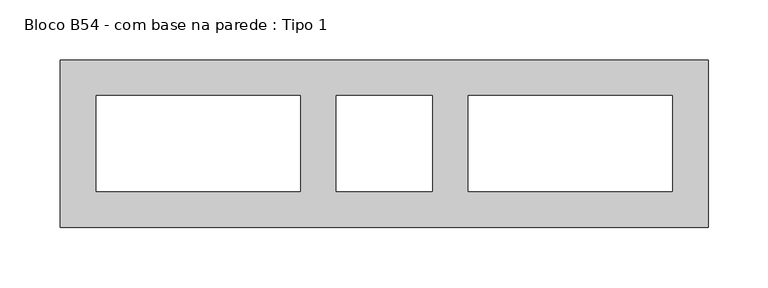
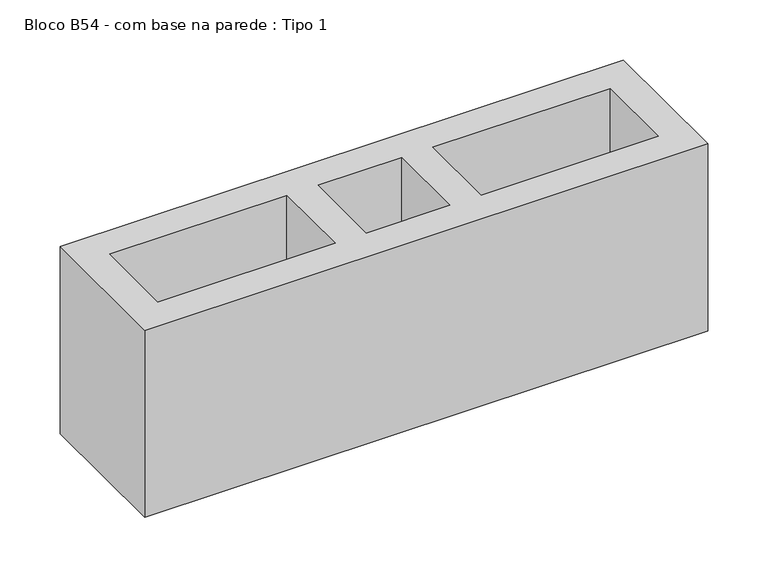
"""IFC4 building model written with IfcOpenShell, lengths in millimetres: proxy geometry, Bloco B54 - com base na parede : Tipo 1."""

from ifc_helpers import new_model, si_unit, origin, origin_with_axes, place, context, project, spatial, polyline, outline, extrude, source, transform, mapped, element, save


def bloco_b54_com_base_na_parede_tipo_1_bb8c27e4(model_context):
    return source(origin(), model_context, "Body", "SweptSolid", [
        extrude(outline(polyline([(320.0, -70.0), (-220.0, -70.0), (-220.0, 70.0), (320.0, 70.0), (320.0, -70.0)]), holes=[polyline([(120.0, -40.0), (290.0, -40.0), (290.0, 40.0), (120.0, 40.0), (120.0, -40.0)]), polyline([(-20.0, -40.0), (-20.0, 40.0), (-190.0, 40.0), (-190.0, -40.0), (-20.0, -40.0)]), polyline([(90.0, -40.0), (90.0, 40.0), (10.0, 40.0), (10.0, -40.0), (90.0, -40.0)])]), origin_with_axes(), (0.0, 0.0, 1.0), 190.0),
    ])


if __name__ == "__main__":
    model = new_model("IFC4")
    model_context = context("Model", 3, world=origin())
    ifc_project = project(units=[si_unit("LENGTHUNIT", "METRE", prefix="MILLI")], contexts=[model_context])
    site = spatial("IfcSite", under=ifc_project)
    building = spatial("IfcBuilding", under=site)
    placement = place(None, origin())
    bloco_b54_com_base_na_parede_tipo_1_shape = bloco_b54_com_base_na_parede_tipo_1_bb8c27e4(model_context)
    element("IfcBuildingElementProxy", 1, Name="Bloco B54 - com base na parede : Tipo 1", ObjectType="Bloco B54 - com base na parede : Tipo 1", at=placement, inside=building, context=model_context, shape_type="MappedRepresentation", body=[
        mapped(bloco_b54_com_base_na_parede_tipo_1_shape, transform((0.0, 0.0, 0.0), x_axis=(1.0, 0.0, 0.0), y_axis=(0.0, 1.0, 0.0), z_axis=(0.0, 0.0, 1.0))),
    ])
    save(model, "model.ifc")

# Revit data of these elements
# Type "Bloco B54 - com base na parede : Tipo 1"
#   SINAPI = ""
#   Assembly Code = ""
